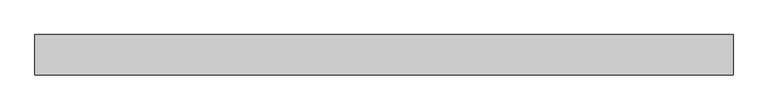
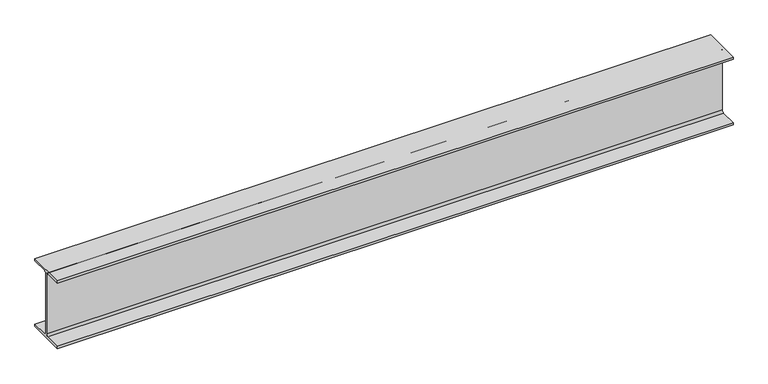
"""IFC4 building model written with IfcOpenShell, lengths in millimetres: beam geometry, Old_Steel Beam_H-KSD3502 : H_SB_ASB_H-200×200x8x12."""

from ifc_helpers import new_model, si_unit, point, frame, frame_2d, origin, place, context, project, spatial, polyline, circle_curve, trimmed, segment, composite_curve, outline, extrude, source, transform, mapped, element, save


def beam_ba2d715d(model_context):
    return source(origin(), model_context, "Body", "SweptSolid", [
        extrude(outline(composite_curve([segment(polyline([(82.5, -141.5), (82.5, -151.7), (-82.5, -151.7), (-82.5, -141.5), (-11.9, -141.5)]), True, "CONTINUOUS"), segment(trimmed(circle_curve(frame_2d((-11.9, -132.6)), 8.9), [point((-11.9, -141.5))], [point((-3.0, -132.6))], True, "CARTESIAN"), True, "CONTINUOUS"), segment(polyline([(-3.0, -132.6), (-3.0, 132.6)]), True, "CONTINUOUS"), segment(trimmed(circle_curve(frame_2d((-11.9, 132.6)), 8.9), [point((-3.0, 132.6))], [point((-11.9, 141.5))], True, "CARTESIAN"), True, "CONTINUOUS"), segment(polyline([(-11.9, 141.5), (-82.5, 141.5), (-82.5, 151.7), (82.5, 151.7), (82.5, 141.5), (11.9, 141.5)]), True, "CONTINUOUS"), segment(trimmed(circle_curve(frame_2d((11.9, 132.6)), 8.9), [point((11.9, 141.5))], [point((3.0, 132.6))], True, "CARTESIAN"), True, "CONTINUOUS"), segment(polyline([(3.0, 132.6), (3.0, -132.6)]), True, "CONTINUOUS"), segment(trimmed(circle_curve(frame_2d((11.9, -132.6)), 8.9), [point((3.0, -132.6))], [point((11.9, -141.5))], True, "CARTESIAN"), True, "CONTINUOUS"), segment(polyline([(11.9, -141.5), (82.5, -141.5)]), True, "CONTINUOUS")], self_intersect=False)), frame((-1273.5795636, 0.0, 0.0), z_axis=(1.0, 0.0, 0.0), x_axis=(0.0, 1.0, 0.0)), (0.0, 0.0, 1.0), 2865.6797009),
    ])


if __name__ == "__main__":
    model = new_model("IFC4")
    model_context = context("Model", 3, world=origin())
    ifc_project = project(units=[si_unit("LENGTHUNIT", "METRE", prefix="MILLI")], contexts=[model_context])
    site = spatial("IfcSite", under=ifc_project)
    building = spatial("IfcBuilding", under=site)
    placement = place(None, origin())
    beam_shape = beam_ba2d715d(model_context)
    element("IfcBeam", 1, ObjectType="Old_Steel Beam_H-KSD3502 : H_SB_ASB_H-200×200x8x12", at=placement, inside=building, context=model_context, shape_type="MappedRepresentation", body=[
        mapped(beam_shape, transform((0.0, 0.0, 0.0), x_axis=(1.0, 0.0, 0.0), y_axis=(0.0, 1.0, 0.0), z_axis=(0.0, 0.0, 1.0))),
    ])
    save(model, "model.ifc")

# Revit data of these elements
# Type "Old_Steel Beam_H-KSD3502 : H_SB_ASB_H-200×200x8x12"
#   Width = 20.0 cm
#   Web Thickness = 0.8 cm
#   Web Fillet = 1.3 cm
#   Warping Constant = 141376.0 cm⁶
#   Torsional Moment of Inertia = 26.2485 cm⁴
#   Torsional Modulus = 1.0 cm³
#   Section Area = 63.53 cm²
#   Plastic Modulus weak axis = 244.0 cm³
#   Plastic Modulus strong axis = 525.0 cm³
#   Perimeter = 1.16 m²/m
#   Nominal Weight = 49.90 kgf/m
#   Moment of Inertia weak axis = 1600.00 cm⁴
#   Moment of Inertia strong axis = 4720.00 cm⁴
#   Height = 20.0 cm
#   Flange Thickness = 1.2 cm
#   Elastic Modulus weak axis = 160.0 cm³
#   Elastic Modulus strong axis = 472.0 cm³
#   Centroid Vertical = 10.0 cm
#   Centroid Horizontal = 10.0 cm
#   Length [instance default] = 1.5240 m
#   Structural Material [instance default] = Steel, 45-345
#   Assembly Code = ""
# Element 1 (IfcBeam, "Old_Steel Beam_H-KSD3502 : H_SB_ASB_H-200×200x8x12")
#   Structural Material = none
# Materials
#   "Steel, 45-345": class "Metal", colour RGB 189 187 185, transparency 0, Description = "Steel 345 MPa", Cost = 0
